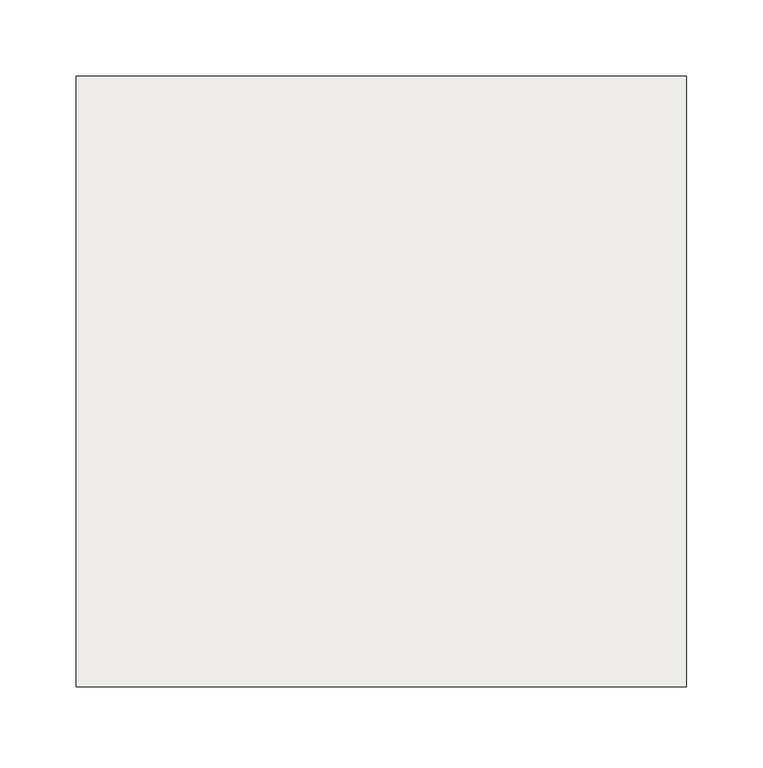
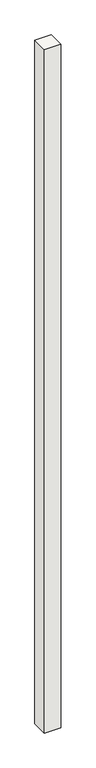
"""IFC4 building model written with IfcOpenShell, lengths in millimetres: slab geometry, NLRS_17_SFO_TLB_funderingspaal geheid beton prefab-AV-MMBPC_gen_rsf : heipaal beton prefab_gen__bxh 400x400."""

from ifc_helpers import new_model, si_unit, frame, origin, place, context, project, spatial, polyline, outline, extrude, source, transform, mapped, element, save


def slab_f6128070(model_context):
    return source(origin(), model_context, "Body", "SweptSolid", [
        extrude(outline(polyline([(200.0, -200.0), (-200.0, -200.0), (-200.0, 200.0), (200.0, 200.0), (200.0, -200.0)])), frame((0.0, 0.0, -20000.0), z_axis=(0.0, 0.0, 1.0), x_axis=(1.0, 0.0, 0.0)), (0.0, 0.0, 1.0), 17610.0),
    ])


if __name__ == "__main__":
    model = new_model("IFC4")
    model_context = context("Model", 3, world=origin())
    ifc_project = project(units=[si_unit("LENGTHUNIT", "METRE", prefix="MILLI")], contexts=[model_context])
    site = spatial("IfcSite", under=ifc_project)
    building = spatial("IfcBuilding", under=site)
    placement = place(None, origin())
    slab_shape = slab_f6128070(model_context)
    element("IfcSlab", 1, ObjectType="NLRS_17_SFO_TLB_funderingspaal geheid beton prefab-AV-MMBPC_gen_rsf : heipaal beton prefab_gen__bxh 400x400", at=placement, inside=building, context=model_context, shape_type="MappedRepresentation", body=[
        mapped(slab_shape, transform((0.0, 0.0, 0.0), x_axis=(1.0, 0.0, 0.0), y_axis=(0.0, 1.0, 0.0), z_axis=(0.0, 0.0, 1.0))),
    ])
    save(model, "model.ifc")

# Revit data of these elements
# Type "NLRS_17_SFO_TLB_funderingspaal geheid beton prefab-AV-MMBPC_gen_rsf : heipaal beton prefab_gen__bxh 400x400"
#   Export Type to IFC As = "IfcPile"
#   Type IfcGUID = "10$Kfo5uPCAOPJEOo5LE_W"
#   Type Comments = "prefab heipaal 400x400"
#   Model = " "
#   Manufacturer = " "
#   Description = "prefab heipaal 400x400"
#   Assembly Code = "17.21"
#   Width = 400 mm
#   Slanted Angle [instance default] = 0.00°
#   NLRS_S_draagvermogen_trek [instance default] = 0.00 kN
#   NLRS_S_draagvermogen_druk [instance default] = 0.00 kN
#   NLRS_C_lengte [instance default] = 1660 mm
#   NLRS_C_hoogte = 400 mm
#   NLRS_C_breedte = 400 mm
#   Height [instance default] = 1660 mm
#   Length [instance default] = 1660 mm
#   Angle [instance default] = 0.00°
#   Slanted [instance default] = 0
#   Structural Material = NLRS_f2_beton prefab_gen_rsf
#   Keynote = ""
# Element 1 (IfcSlab, "NLRS_17_SFO_TLB_funderingspaal geheid beton prefab-AV-MMBPC_gen_rsf : heipaal beton prefab_gen__bxh 400x400")
#   NLRS_C_lengte = 17610 mm
#   Height = 17610 mm
#   Length = 17610 mm
#   Materials on its faces: "NLRS_f2_beton prefab_gen_rsf"
# Materials
#   "NLRS_f2_beton prefab_gen_rsf": class "F - Niet gebakken kunststeen", colour RGB 129 133 118, transparency 0, Keynote = "f2", Manufacturer = "Revit Standards Foundation", URL = "www.revitstandards.org", Description = "beton prefab", Cost = 0
